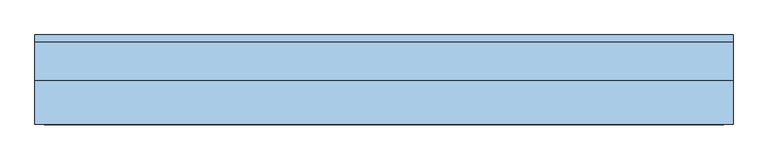
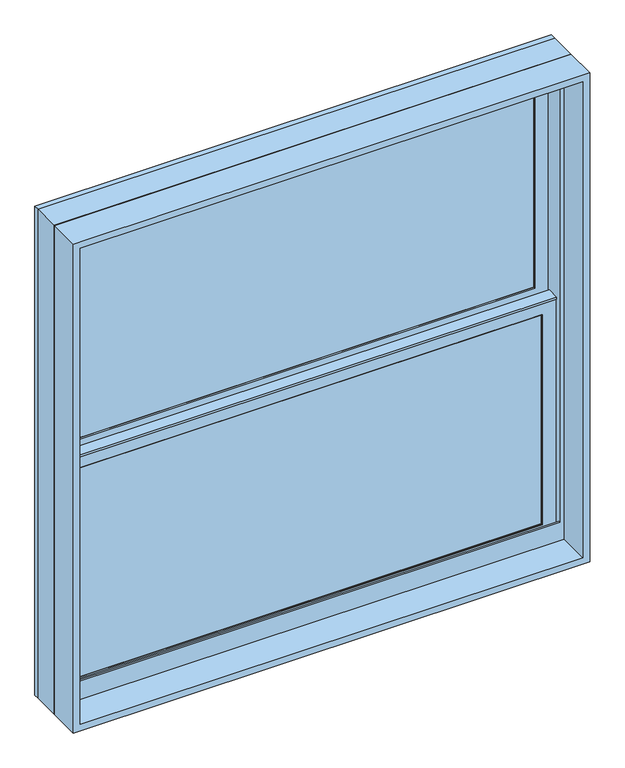
"""IFC4 building model written with IfcOpenShell, lengths in millimetres: window geometry, Window-Double_Hung-Marvin-Essential : ESDH4040."""

from ifc_helpers import new_model, si_unit, frame, origin, place, context, project, spatial, polyline, outline, extrude, faceted_brep, source, transform, mapped, element, save


def window_c6c91ca5(model_context):
    return source(origin(), model_context, "Body", "SolidModel", [
        extrude(outline(polyline([(191.5583333, 20.6375), (191.5583333, 15.875), (172.5083333, 15.875), (172.5083333, 20.6375), (191.5583333, 20.6375)])), frame((0.0, 0.0, 1289.05), z_axis=(0.0, 0.0, 1.0), x_axis=(1.0, 0.0, 0.0)), (0.0, 0.0, 1.0), 527.05),
        extrude(outline(polyline([(-172.5083333, 20.6375), (-172.5083333, 15.875), (-191.5583333, 15.875), (-191.5583333, 20.6375), (-172.5083333, 20.6375)])), frame((0.0, 0.0, 1289.05), z_axis=(0.0, 0.0, 1.0), x_axis=(1.0, 0.0, 0.0)), (0.0, 0.0, 1.0), 527.05),
        extrude(outline(polyline([(546.1, 20.6375), (546.1, 15.875), (-546.1, 15.875), (-546.1, 20.6375), (546.1, 20.6375)])), frame((0.0, 0.0, 1543.05), z_axis=(0.0, 0.0, 1.0), x_axis=(1.0, 0.0, 0.0)), (0.0, 0.0, 1.0), 19.05),
        extrude(outline(polyline([(-191.5583333, 46.83125), (-191.5583333, 51.59375), (-172.5083333, 51.59375), (-172.5083333, 46.83125), (-191.5583333, 46.83125)])), frame((0.0, 0.0, 1854.2), z_axis=(0.0, 0.0, 1.0), x_axis=(1.0, 0.0, 0.0)), (0.0, 0.0, 1.0), 527.05),
        extrude(outline(polyline([(172.5083333, 46.83125), (172.5083333, 51.59375), (191.5583333, 51.59375), (191.5583333, 46.83125), (172.5083333, 46.83125)])), frame((0.0, 0.0, 1854.2), z_axis=(0.0, 0.0, 1.0), x_axis=(1.0, 0.0, 0.0)), (0.0, 0.0, 1.0), 527.05),
        extrude(outline(polyline([(-546.1, 46.83125), (-546.1, 51.59375), (546.1, 51.59375), (546.1, 46.83125), (-546.1, 46.83125)])), frame((0.0, 0.0, 2108.2), z_axis=(0.0, 0.0, 1.0), x_axis=(1.0, 0.0, 0.0)), (0.0, 0.0, 1.0), 19.05),
        extrude(outline(polyline([(191.5583333, 20.6375), (172.5083333, 20.6375), (172.5083333, 25.4), (191.5583333, 25.4), (191.5583333, 20.6375)])), frame((0.0, 0.0, 1289.05), z_axis=(0.0, 0.0, 1.0), x_axis=(1.0, 0.0, 0.0)), (0.0, 0.0, 1.0), 527.05),
        extrude(outline(polyline([(-172.5083333, 20.6375), (-191.5583333, 20.6375), (-191.5583333, 25.4), (-172.5083333, 25.4), (-172.5083333, 20.6375)])), frame((0.0, 0.0, 1289.05), z_axis=(0.0, 0.0, 1.0), x_axis=(1.0, 0.0, 0.0)), (0.0, 0.0, 1.0), 527.05),
        extrude(outline(polyline([(546.1, 20.6375), (-546.1, 20.6375), (-546.1, 25.4), (546.1, 25.4), (546.1, 20.6375)])), frame((0.0, 0.0, 1543.05), z_axis=(0.0, 0.0, 1.0), x_axis=(1.0, 0.0, 0.0)), (0.0, 0.0, 1.0), 19.05),
        extrude(outline(polyline([(-191.5583333, 56.35625), (-172.5083333, 56.35625), (-172.5083333, 51.59375), (-191.5583333, 51.59375), (-191.5583333, 56.35625)])), frame((0.0, 0.0, 1854.2), z_axis=(0.0, 0.0, 1.0), x_axis=(1.0, 0.0, 0.0)), (0.0, 0.0, 1.0), 527.05),
        extrude(outline(polyline([(172.5083333, 56.35625), (191.5583333, 56.35625), (191.5583333, 51.59375), (172.5083333, 51.59375), (172.5083333, 56.35625)])), frame((0.0, 0.0, 1854.2), z_axis=(0.0, 0.0, 1.0), x_axis=(1.0, 0.0, 0.0)), (0.0, 0.0, 1.0), 527.05),
        extrude(outline(polyline([(-546.1, 56.35625), (546.1, 56.35625), (546.1, 51.59375), (-546.1, 51.59375), (-546.1, 56.35625)])), frame((0.0, 0.0, 2108.2), z_axis=(0.0, 0.0, 1.0), x_axis=(1.0, 0.0, 0.0)), (0.0, 0.0, 1.0), 19.05),
        faceted_brep([(-573.0875, 5.6780605, 1846.1351748), (-573.0875, 5.6780605, 1841.5), (573.0875, 5.6780605, 1841.5), (573.0875, 5.6780605, 1846.1351748), (-573.0875, 34.8118605, 1846.1351748), (573.0875, 34.8118605, 1846.1351748), (573.0875, 34.8118605, 1841.5), (-573.0875, 34.8118605, 1841.5), (-573.0875, 30.1625, 1841.5), (-573.0875, 30.1625, 1262.0625), (-573.0875, 8.9241104, 1262.0625), (-573.0875, 8.9241104, 1841.5), (573.0875, 8.9241104, 1841.5), (573.0875, 30.1625, 1841.5), (573.0875, 8.9241104, 1262.0625), (573.0875, 30.1625, 1262.0625), (-557.2034752, 11.90625, 1827.2034752), (-557.2034752, 30.1625, 1827.2034752), (557.2034752, 30.1625, 1827.2034752), (557.2034752, 11.90625, 1827.2034752), (-540.54375, 10.4662439, 1810.54375), (-540.54375, 11.90625, 1810.54375), (540.54375, 11.90625, 1810.54375), (540.54375, 10.4662439, 1810.54375), (542.0858834, 8.9241104, 1812.0858834), (-542.0858834, 8.9241104, 1812.0858834), (557.2034752, 30.1625, 1277.9465248), (557.2034752, 11.90625, 1277.9465248), (540.54375, 11.90625, 1294.60625), (540.54375, 10.4662439, 1294.60625), (542.0858834, 8.9241104, 1293.0641166), (-557.2034752, 30.1625, 1277.9465248), (-557.2034752, 11.90625, 1277.9465248), (-540.54375, 11.90625, 1294.60625), (-540.54375, 10.4662439, 1294.60625), (-542.0858834, 8.9241104, 1293.0641166)], [[[0, 1, 2, 3]], [[4, 5, 6, 7]], [[1, 0, 4, 7, 8, 9, 10, 11]], [[2, 1, 11, 12]], [[7, 6, 13, 8]], [[3, 2, 12, 14, 15, 13, 6, 5]], [[0, 3, 5, 4]], [[16, 17, 18, 19]], [[20, 21, 22, 23]], [[20, 23, 24, 25]], [[19, 18, 26, 27]], [[23, 22, 28, 29]], [[24, 23, 29, 30]], [[27, 26, 31, 32]], [[29, 28, 33, 34]], [[30, 29, 34, 35]], [[15, 14, 10, 9]], [[15, 9, 8, 13], [18, 17, 31, 26]], [[17, 16, 32, 31]], [[16, 19, 27, 32], [22, 21, 33, 28]], [[21, 20, 34, 33]], [[20, 25, 35, 34]], [[10, 14, 12, 11], [25, 24, 30, 35]]]),
        extrude(outline(polyline([(38.5955581, 1827.2125), (33.5778968, 1827.2125), (33.5778968, 1828.8), (39.9405976, 1828.8), (39.9405976, 1827.2125), (61.515625, 1827.2125), (47.6307501, 1823.8975159), (38.5955581, 1823.8975159), (38.5955581, 1827.2125)])), frame((-573.0875, 0.0, 0.0), z_axis=(1.0, 0.0, 0.0), x_axis=(0.0, 1.0, 0.0)), (0.0, 0.0, 1.0), 1146.175),
        faceted_brep([(603.25, 0.0, 1231.9), (603.25, 0.0, 2438.4), (-603.25, 0.0, 2438.4), (-603.25, 0.0, 1231.9), (577.05625, 0.0, 1293.01875), (-577.05625, 0.0, 1293.01875), (-577.05625, 0.0, 2412.20625), (577.05625, 0.0, 2412.20625), (577.05625, 3.96875, 1231.9), (-577.05625, 3.96875, 1231.9), (-577.05625, 3.96875, 1293.01875), (577.05625, 3.96875, 1293.01875), (-603.25, 65.6828125, 1231.9), (-577.05625, 65.6828125, 1231.9), (577.05625, 65.6828125, 1231.9), (603.25, 65.6828125, 1231.9), (-603.25, 65.6828125, 2438.4), (603.25, 65.6828125, 2438.4), (577.05625, 65.6828125, 2412.20625), (-577.05625, 65.6828125, 2412.20625)], [[[0, 1, 2, 3], [4, 5, 6, 7]], [[8, 9, 10, 11]], [[5, 4, 11, 10]], [[0, 3, 12, 13, 9, 8, 14, 15]], [[13, 12, 16, 17, 15, 14, 18, 19]], [[13, 19, 6, 5, 10, 9]], [[7, 6, 19, 18]], [[18, 14, 8, 11, 4, 7]], [[1, 0, 15, 17]], [[2, 1, 17, 16]], [[3, 2, 16, 12]]]),
        faceted_brep([(577.05625, 30.1625, 1835.15), (575.46875, 30.1625, 1835.15), (575.46875, 30.1625, 1256.2544613), (577.05625, 30.1625, 1256.2544613), (-575.46875, 30.1625, 1835.15), (-577.05625, 30.1625, 1835.15), (-577.05625, 30.1625, 1256.2544613), (-575.46875, 30.1625, 1256.2544613), (575.46875, 63.5, 1835.15), (577.05625, 63.5, 1835.15), (577.05625, 63.5, 1249.7743077), (575.46875, 63.5, 1249.7743077), (-577.05625, 63.5, 1835.15), (-575.46875, 63.5, 1835.15), (-575.46875, 63.5, 1249.7743077), (-577.05625, 63.5, 1249.7743077), (588.3108932, 3.96875, 1261.3460105), (588.3108932, 3.96875, 1231.9), (588.3108932, 65.6828125, 1231.9), (588.3108932, 65.6828125, 1249.350012), (-588.3108932, 3.96875, 1231.9), (-588.3108932, 3.96875, 1261.3460105), (-588.3108932, 65.6828125, 1249.350012), (-588.3108932, 65.6828125, 1231.9), (588.3108932, 78.58125, 1246.8428097), (-588.3108932, 78.58125, 1246.8428097), (-586.2971252, 68.2348864, 1248.8539391), (-568.33135, 68.2348864, 1248.8539391), (-568.33135, 65.6828125, 1249.350012), (568.33135, 65.6828125, 1249.350012), (568.33135, 68.2348864, 1248.8539391), (586.2971252, 68.2348864, 1248.8539391), (-603.25, 65.6828125, 1231.9), (-603.25, 78.5948249, 1231.9), (603.25, 78.5948249, 1231.9), (603.25, 65.6828125, 1231.9), (-603.25, 78.58125, 2438.4), (603.25, 78.58125, 2438.4), (588.3108932, 78.58125, 2423.4608932), (-588.3108932, 78.58125, 2423.4608932), (-603.25, 65.6828125, 2438.4), (-586.2971252, 68.2348864, 2421.4471252), (586.2971252, 68.2348864, 2421.4471252), (568.33135, 68.2348864, 2403.48135), (-568.33135, 68.2348864, 2403.48135), (-568.33135, 65.6828125, 2403.48135), (568.33135, 65.6828125, 2403.48135), (603.25, 65.6828125, 2438.4)], [[[0, 1, 2, 3]], [[4, 5, 6, 7]], [[8, 9, 10, 11]], [[12, 13, 14, 15]], [[1, 8, 11, 2]], [[9, 0, 3, 10]], [[1, 0, 9, 8]], [[5, 4, 13, 12]], [[5, 12, 15, 6]], [[13, 4, 7, 14]], [[16, 17, 18, 19]], [[20, 21, 22, 23]], [[24, 25, 26, 27, 28, 22, 21, 16, 19, 29, 30, 31], [3, 2, 11, 10], [7, 6, 15, 14]], [[17, 16, 21, 20]], [[17, 20, 23, 32, 33, 34, 35, 18]], [[34, 33, 36, 37], [25, 24, 38, 39]], [[33, 32, 40, 36]], [[39, 41, 26, 25]], [[41, 42, 31, 30, 43, 44, 27, 26]], [[44, 45, 28, 27]], [[40, 32, 23, 22, 28, 45, 46, 29, 19, 18, 35, 47]], [[36, 40, 47, 37]], [[39, 38, 42, 41]], [[44, 43, 46, 45]], [[34, 37, 47, 35]], [[42, 38, 24, 31]], [[46, 43, 30, 29]]]),
        extrude(outline(polyline([(553.24375, 11.90625), (-553.24375, 11.90625), (-553.24375, 15.08125), (553.24375, 15.08125), (553.24375, 11.90625)])), frame((0.0, 0.0, 1281.90625), z_axis=(0.0, 0.0, 1.0), x_axis=(1.0, 0.0, 0.0)), (0.0, 0.0, 1.0), 541.3375),
        extrude(outline(polyline([(553.24375, 42.8625), (-553.24375, 42.8625), (-553.24375, 46.0375), (553.24375, 46.0375), (553.24375, 42.8625)])), frame((0.0, 0.0, 1847.05625), z_axis=(0.0, 0.0, 1.0), x_axis=(1.0, 0.0, 0.0)), (0.0, 0.0, 1.0), 541.3375),
        faceted_brep([(-540.54375, 31.194477, 1810.54375), (-542.0858834, 32.7366104, 1812.0858834), (542.0858834, 32.7366104, 1812.0858834), (540.54375, 31.194477, 1810.54375), (-540.54375, 30.1625, 1810.54375), (540.54375, 30.1625, 1810.54375), (-573.0875, 32.7366104, 1843.0875), (-573.0875, 30.1625, 1843.0875), (573.0875, 30.1625, 1843.0875), (573.0875, 32.7366104, 1843.0875), (542.0858834, 32.7366104, 1293.0641166), (540.54375, 31.194477, 1294.60625), (540.54375, 30.1625, 1294.60625), (573.0875, 30.1625, 1262.0625), (573.0875, 32.7366104, 1262.0625), (-542.0858834, 32.7366104, 1293.0641166), (-540.54375, 31.194477, 1294.60625), (-540.54375, 30.1625, 1294.60625), (-573.0875, 30.1625, 1262.0625), (-573.0875, 32.7366104, 1262.0625)], [[[0, 1, 2, 3]], [[4, 0, 3, 5]], [[6, 7, 8, 9]], [[3, 2, 10, 11]], [[5, 3, 11, 12]], [[9, 8, 13, 14]], [[11, 10, 15, 16]], [[12, 11, 16, 17]], [[14, 13, 18, 19]], [[9, 14, 19, 6], [1, 15, 10, 2]], [[16, 15, 1, 0]], [[17, 16, 0, 4]], [[7, 18, 13, 8], [5, 12, 17, 4]], [[19, 18, 7, 6]]]),
        faceted_brep([(-557.2034752, 42.8625, 2392.3534752), (-557.2034752, 61.11875, 2392.3534752), (557.2034752, 61.11875, 2392.3534752), (557.2034752, 42.8625, 2392.3534752), (-540.54375, 41.4224939, 2375.69375), (-540.54375, 42.8625, 2375.69375), (540.54375, 42.8625, 2375.69375), (540.54375, 41.4224939, 2375.69375), (-542.0858834, 39.8803604, 2377.2358834), (542.0858834, 39.8803604, 2377.2358834), (-573.0875, 61.11875, 2408.2375), (-573.0875, 39.8803604, 2408.2375), (573.0875, 39.8803604, 2408.2375), (573.0875, 61.11875, 2408.2375), (557.2034752, 61.11875, 1843.0965248), (557.2034752, 42.8625, 1843.0965248), (540.54375, 42.8625, 1859.75625), (540.54375, 41.4224939, 1859.75625), (542.0858834, 39.8803604, 1858.2141166), (573.0875, 39.8803604, 1827.2125), (573.0875, 61.11875, 1827.2125), (-557.2034752, 61.11875, 1843.0965248), (-557.2034752, 42.8625, 1843.0965248), (-540.54375, 42.8625, 1859.75625), (-540.54375, 41.4224939, 1859.75625), (-542.0858834, 39.8803604, 1858.2141166), (-573.0875, 39.8803604, 1827.2125), (-573.0875, 61.11875, 1827.2125)], [[[0, 1, 2, 3]], [[4, 5, 6, 7]], [[8, 4, 7, 9]], [[10, 11, 12, 13]], [[3, 2, 14, 15]], [[7, 6, 16, 17]], [[9, 7, 17, 18]], [[13, 12, 19, 20]], [[15, 14, 21, 22]], [[17, 16, 23, 24]], [[18, 17, 24, 25]], [[20, 19, 26, 27]], [[13, 20, 27, 10], [1, 21, 14, 2]], [[22, 21, 1, 0]], [[3, 15, 22, 0], [5, 23, 16, 6]], [[24, 23, 5, 4]], [[25, 24, 4, 8]], [[11, 26, 19, 12], [9, 18, 25, 8]], [[27, 26, 11, 10]]]),
        faceted_brep([(-573.0875, 61.11875, 1827.2125), (-573.0875, 63.6928604, 1827.2125), (573.0875, 63.6928604, 1827.2125), (573.0875, 61.11875, 1827.2125), (-540.54375, 62.150727, 1859.75625), (-540.54375, 61.11875, 1859.75625), (540.54375, 61.11875, 1859.75625), (540.54375, 62.150727, 1859.75625), (-542.0858834, 63.6928604, 1858.2141166), (542.0858834, 63.6928604, 1858.2141166), (573.0875, 63.6928604, 2408.2375), (573.0875, 61.11875, 2408.2375), (540.54375, 61.11875, 2375.69375), (540.54375, 62.150727, 2375.69375), (542.0858834, 63.6928604, 2377.2358834), (-573.0875, 63.6928604, 2408.2375), (-573.0875, 61.11875, 2408.2375), (-540.54375, 61.11875, 2375.69375), (-540.54375, 62.150727, 2375.69375), (-542.0858834, 63.6928604, 2377.2358834)], [[[0, 1, 2, 3]], [[4, 5, 6, 7]], [[8, 4, 7, 9]], [[3, 2, 10, 11]], [[7, 6, 12, 13]], [[9, 7, 13, 14]], [[11, 10, 15, 16]], [[13, 12, 17, 18]], [[14, 13, 18, 19]], [[16, 15, 1, 0]], [[3, 11, 16, 0], [5, 17, 12, 6]], [[18, 17, 5, 4]], [[19, 18, 4, 8]], [[1, 15, 10, 2], [9, 14, 19, 8]]]),
        extrude(outline(polyline([(553.24375, 26.19375), (-553.24375, 26.19375), (-553.24375, 30.1625), (553.24375, 30.1625), (553.24375, 26.19375)])), frame((0.0, 0.0, 1281.90625), z_axis=(0.0, 0.0, 1.0), x_axis=(1.0, 0.0, 0.0)), (0.0, 0.0, 1.0), 541.3375),
        extrude(outline(polyline([(553.24375, 57.15), (-553.24375, 57.15), (-553.24375, 61.11875), (553.24375, 61.11875), (553.24375, 57.15)])), frame((0.0, 0.0, 1847.05625), z_axis=(0.0, 0.0, 1.0), x_axis=(1.0, 0.0, 0.0)), (0.0, 0.0, 1.0), 541.3375),
        extrude(outline(polyline([(2438.4, 603.25), (2438.4, -603.25), (1231.9, -603.25), (1231.9, 603.25), (2438.4, 603.25)]), holes=[polyline([(2422.525, 587.375), (1247.775, 587.375), (1247.775, -587.375), (2422.525, -587.375), (2422.525, 587.375)])]), frame((0.0, -76.2, 0.0), z_axis=(0.0, 1.0, 0.0), x_axis=(0.0, 0.0, 1.0)), (0.0, 0.0, 1.0), 75.40625),
    ])


if __name__ == "__main__":
    model = new_model("IFC4")
    model_context = context("Model", 3, world=origin())
    ifc_project = project(units=[si_unit("LENGTHUNIT", "METRE", prefix="MILLI")], contexts=[model_context])
    site = spatial("IfcSite", under=ifc_project)
    building = spatial("IfcBuilding", under=site)
    placement = place(None, origin())
    window_shape = window_c6c91ca5(model_context)
    element("IfcWindow", 1, ObjectType="Window-Double_Hung-Marvin-Essential : ESDH4040", at=placement, inside=building, context=model_context, shape_type="MappedRepresentation", body=[
        mapped(window_shape, transform((0.0, 0.0, 0.0), x_axis=(1.0, 0.0, 0.0), y_axis=(0.0, 1.0, 0.0), z_axis=(0.0, 0.0, 1.0))),
    ])
    save(model, "model.ifc")

# Revit data of these elements
# Type "Window-Double_Hung-Marvin-Essential : ESDH4040"
#   Type Mark = "53"
#   Window Type = "Essential Double Hung"
#   Product data url = "https://bimobject.com/marvin-windows-and-doors/product/marvin-dhwau"
#   Product Guid = "c4a96547-874c-4385-91dc-a058adc19d98"
#   Frame = "All Ultrex"
#   Egress Window = "No"
#   URL = "www.marvin.com"
#   Model = "ESDH4040"
#   Manufacturer = "Marvin Windows and Doors"
#   Label Egress = ""
#   Glass Type = "IG Low E II with Argon"
#   Design Pressure = "DP50"
#   Description = "4848 DBHG"
#   Analytic Construction = "<None>"
#   Prairie Corner Width = 0' - 4"
#   Prairie Corner Height = 0' - 4"
#   Egress Width = 3' - 8 9/16"
#   Egress Height = 1' - 7 27/128"
#   Rough Width = 4' - 0"
#   Rough Height = 4' - 0"
#   Nominal Width = 4' - 0"
#   Nominal Height = 4' - 0"
#   Inset to Installation Flange [instance default] = 0' - 1"
#   Height = 3' - 11 1/2"
#   Egress Area = 5.94505 SF
#   Default Head Height = 8' - 0"
#   Width = 3' - 11 1/2"
#   Daylight Area = 12.0076 SF
#   DLO Width = 3' - 6 9/16"
#   DLO Height = 1' - 8 5/16"
#   Muntins Top Sash = yes
#   Lites Wide Top Sash = 3
#   Lites Wide Bottom Sash = 3
#   Lites High Top Sash = 2
#   Lites High Bottom Sash = 2
#   Lite Cut Prairie 9 = no
#   Lite Cut HV Grid = yes
#   Muntins Bottom Sash = yes
#   Label Visibility = no
#   Jamb Extension Visibility = yes
#   Edition number = 1
#   Interior Material = Ultrex-Marvin-Stonewhite
#   Glazing Material = Glass-Marvin-IG Low E II with Argon
#   Cladding Material = Ultrex-Marvin-Pebblegray
#   Wall Closure = (empty or 0)
#   Assembly Code = ""
# Element 1 (IfcWindow, "Window-Double_Hung-Marvin-Essential : ESDH4040")
#   Materials on its faces: "Ultrex-Marvin-Pebblegray", "Ultrex-Marvin-Stonewhite", "Glass-Marvin-IG Low E II with Argon"
# Materials
#   "Ultrex-Marvin-Stonewhite": class "Paint", colour RGB 250 251 245, transparency 0
#   "Glass-Marvin-IG Low E II with Argon": class "Glass", colour RGB 0 128 192, transparency 0.85
#   "Ultrex-Marvin-Pebblegray": class "Paint", colour RGB 189 185 173, transparency 0
